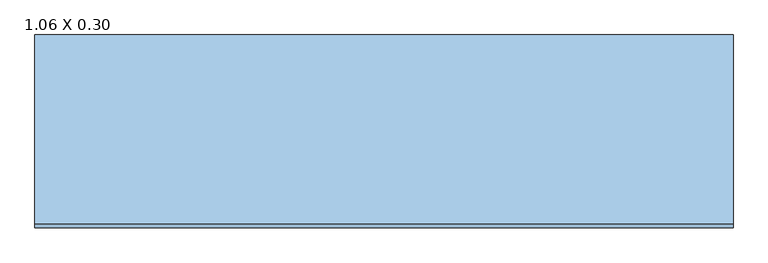
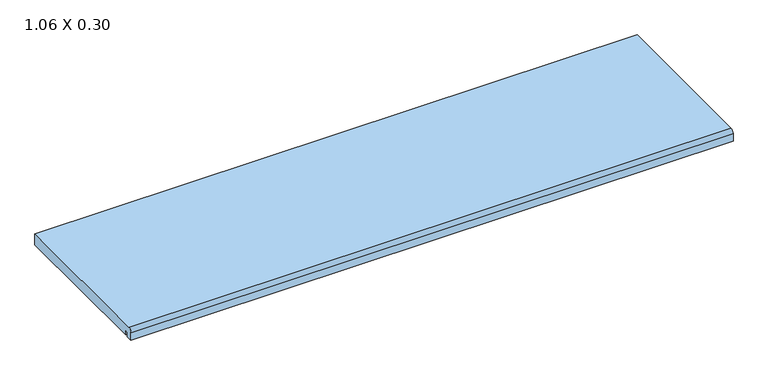
"""IFC4 building model written with IfcOpenShell, lengths in millimetres: window geometry, .CC_ND 300_PEDRA_PEITORIL RETO : 1.06 X 0.30."""

from ifc_helpers import new_model, si_unit, point, frame, frame_2d, origin, place, context, project, spatial, polyline, circle_curve, trimmed, segment, composite_curve, outline, extrude, source, transform, mapped, element, save


def window_1_06_x_0_30_49639a84(model_context):
    return source(origin(), model_context, "Body", "SweptSolid", [
        extrude(outline(composite_curve([segment(polyline([(-132.5083081, 1480.0), (-132.5083081, 1488.1993124), (-137.2619526, 1488.1993124), (-137.2619526, 1480.0), (-148.0, 1480.0), (-148.0, 1493.3808343)]), True, "CONTINUOUS"), segment(trimmed(circle_curve(frame_2d((-141.3808343, 1493.3808343)), 6.6191657), [point((-148.0, 1493.3808343))], [point((-141.3808343, 1500.0))], False, "CARTESIAN"), True, "CONTINUOUS"), segment(polyline([(-141.3808343, 1500.0), (145.0, 1500.0), (145.0, 1480.0), (-132.5083081, 1480.0)]), True, "CONTINUOUS")], self_intersect=False)), frame((-530.0, 0.0, 0.0), z_axis=(1.0, 0.0, 0.0), x_axis=(0.0, 1.0, 0.0)), (0.0, 0.0, 1.0), 1060.0),
    ])


if __name__ == "__main__":
    model = new_model("IFC4")
    model_context = context("Model", 3, world=origin())
    ifc_project = project(units=[si_unit("LENGTHUNIT", "METRE", prefix="MILLI")], contexts=[model_context])
    site = spatial("IfcSite", under=ifc_project)
    building = spatial("IfcBuilding", under=site)
    placement = place(None, origin())
    window_1_06_x_0_30_shape = window_1_06_x_0_30_49639a84(model_context)
    element("IfcWindow", 1, ObjectType=".CC_ND 300_PEDRA_PEITORIL RETO : 1.06 X 0.30", at=placement, inside=building, context=model_context, shape_type="MappedRepresentation", body=[
        mapped(window_1_06_x_0_30_shape, transform((0.0, 0.0, 0.0), x_axis=(1.0, 0.0, 0.0), y_axis=(0.0, 1.0, 0.0), z_axis=(0.0, 0.0, 1.0))),
    ])
    save(model, "model.ifc")

# Revit data of these elements
# Type ".CC_ND 300_PEDRA_PEITORIL RETO : 1.06 X 0.30"
#   Type Mark = "68"
#   Largura da pedra [instance default] = 0.26 m
#   Extensão interior peitoril [instance default] = 0.03 m
#   Extensão exterior peitoril [instance default] = 0.03 m
#   Espessura = 0.02 m
#   Comprimento = 1.06 m
#   Altura-padrão do peitoril = 1.48 m
#   Peitoril = .GRANITO_BRANCO_ITAUNAS
#   Rough Width = 0
#   Rough Height = 0
#   Height = 0
#   Wall Closure = (empty or 0)
#   Width = 0
# Element 1 (IfcWindow, ".CC_ND 300_PEDRA_PEITORIL RETO : 1.06 X 0.30")
#   Largura da pedra = 0.293 m
#   Extensão interior peitoril = 0.027 m
#   Materials on its faces: ".GRANITO_BRANCO_ITAUNAS"
# Materials
#   ".GRANITO_BRANCO_ITAUNAS": class ".CC_PEDRA REVEST.", colour RGB 202 195 174, transparency 0, Description = "Revestimento em granito", Cost = 0
